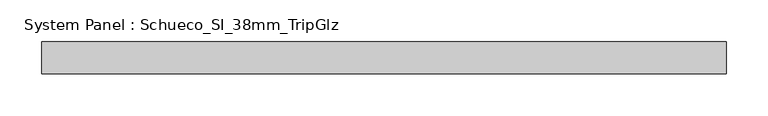
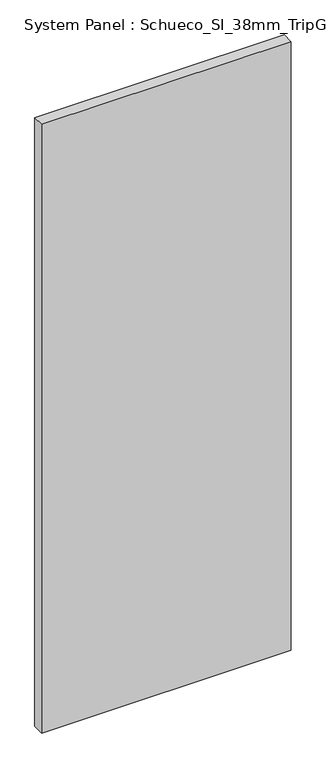
"""IFC4 building model written with IfcOpenShell, lengths in millimetres: plate geometry, System Panel : Schueco_SI_38mm_TripGlz."""

from ifc_helpers import new_model, si_unit, origin, origin_with_axes, place, context, project, spatial, polyline, outline, extrude, source, transform, mapped, element, save


def system_panel_schueco_si_38mm_tripglz_8364d7db(model_context):
    return source(origin(), model_context, "Body", "SweptSolid", [
        extrude(outline(polyline([(409.0, -38.0), (-409.0, -38.0), (-409.0, 0.0), (409.0, 0.0), (409.0, -38.0)])), origin_with_axes(), (0.0, 0.0, 1.0), 2108.0),
    ])


if __name__ == "__main__":
    model = new_model("IFC4")
    model_context = context("Model", 3, world=origin())
    ifc_project = project(units=[si_unit("LENGTHUNIT", "METRE", prefix="MILLI")], contexts=[model_context])
    site = spatial("IfcSite", under=ifc_project)
    building = spatial("IfcBuilding", under=site)
    placement = place(None, origin())
    system_panel_schueco_si_38mm_tripglz_shape = system_panel_schueco_si_38mm_tripglz_8364d7db(model_context)
    element("IfcPlate", 1, ObjectType="System Panel : Schueco_SI_38mm_TripGlz", at=placement, inside=building, context=model_context, shape_type="MappedRepresentation", body=[
        mapped(system_panel_schueco_si_38mm_tripglz_shape, transform((0.0, 0.0, 0.0), x_axis=(1.0, 0.0, 0.0), y_axis=(0.0, 1.0, 0.0), z_axis=(0.0, 0.0, 1.0))),
    ])
    save(model, "model.ifc")

# Revit data of these elements
# Type "System Panel : Schueco_SI_38mm_TripGlz"
#   Model = "Triple glazing 38mm"
# Element 1 (IfcPlate, "System Panel : Schueco_SI_38mm_TripGlz")
#   Materials on its faces: "Glass"
# Materials
#   "Glass": class "Glass", colour RGB 128 128 255, transparency 0.75, Description = "Soda Lime Glass", Cost = 0
